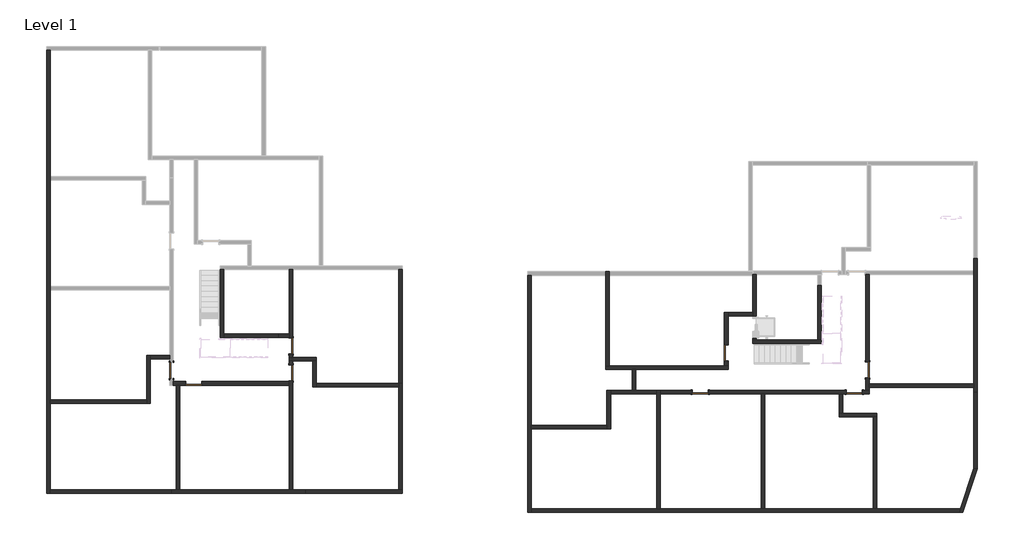
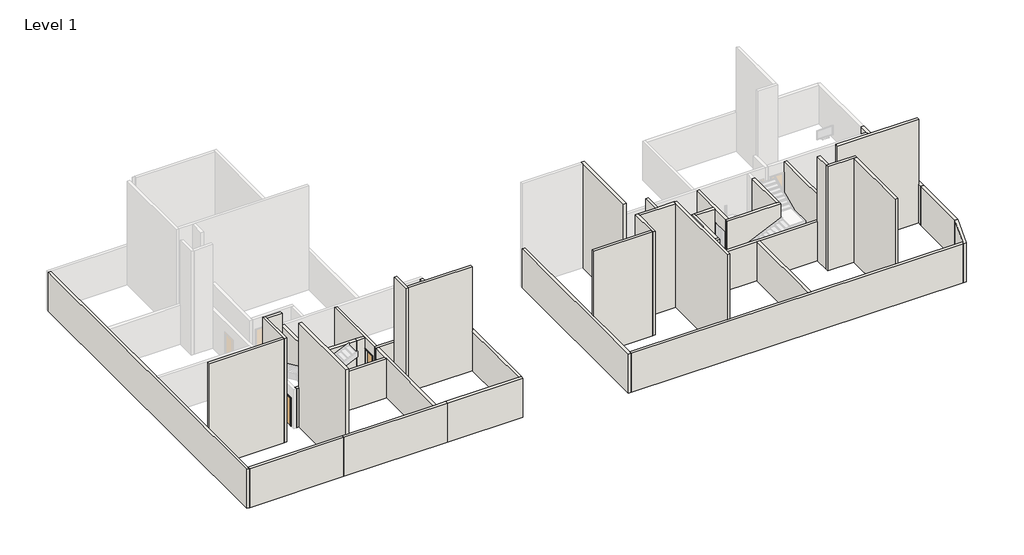
# One storey, part 1 of 2: 43 walls, 8 doors.
# Revit data of these elements (continued)
# Room, not placed, phase "New Construction", upper offset 0 cm, lower offset 0 cm
#   Number = "5"
#   Name = "Room"
# Room, not placed, phase "New Construction", upper offset 0 cm, lower offset 0 cm
#   Number = "6"
#   Name = "Room"
# Room at (-9476.825, 5160.6) mm, phase "New Construction", upper level "Level 1", upper offset 243.84 cm, lower offset 0 cm
#   Number = "124"
#   Name = "Room"
# Room, not placed, phase "New Construction", upper offset 0 cm, lower offset 0 cm
#   Number = "34"
#   Name = "Room"
# Room, not placed, phase "New Construction", upper offset 0 cm, lower offset 0 cm
#   Number = "35"
#   Name = "Room"
# Room, not placed, phase "New Construction", upper offset 0 cm, lower offset 0 cm
#   Number = "9"
#   Name = "Room"
# Room, not placed, phase "New Construction", upper offset 0 cm, lower offset 0 cm
#   Number = "10"
#   Name = "Room"
# Room, not placed, phase "New Construction", upper offset 0 cm, lower offset 0 cm
#   Number = "125"
#   Name = "Room"
# Room, not placed, phase "New Construction", upper offset 0 cm, lower offset 0 cm
#   Number = "126"
#   Name = "Room"
# Room, not placed, phase "New Construction", upper offset 0 cm, lower offset 0 cm
#   Number = "127"
#   Name = "Room"
# Room, not placed, phase "New Construction", upper offset 0 cm, lower offset 0 cm
#   Number = "128"
#   Name = "Room"
# Room, not placed, phase "New Construction", upper offset 0 cm, lower offset 0 cm
#   Number = "129"
#   Name = "Room"
# Room, not placed, phase "New Construction", upper offset 0 cm, lower offset 0 cm
#   Number = "91"
#   Name = "Room"
# Room at (-20321.225, 11202.195) mm, phase "New Construction", upper level "Level 1", upper offset 243.84 cm, lower offset 0 cm
#   Number = "130"
#   Name = "Room"
# Room at (-5594.466, -7580.79) mm, phase "New Construction", upper level "Level 1", upper offset 243.84 cm, lower offset 0 cm
#   Number = "131"
#   Name = "Room"
# Room at (-4954.966, -1430.614) mm, phase "New Construction", upper level "Level 1", upper offset 243.84 cm, lower offset 0 cm
#   Number = "132"
#   Name = "Room"
# Room at (-12237.947, 10302.814) mm, phase "New Construction", upper level "Level 1", upper offset 243.84 cm, lower offset 0 cm
#   Number = "133"
#   Name = "Room"
# Room, not placed, phase "New Construction", upper offset 0 cm, lower offset 0 cm
#   Number = ""
#   Name = ""
# Room, not placed, phase "New Construction", upper offset 0 cm, lower offset 0 cm
#   Number = "70"
#   Name = "Room"
# Room, not placed, phase "New Construction", upper offset 0 cm, lower offset 0 cm
#   Number = "71"
#   Name = "Room"
# Room, not placed, phase "New Construction", upper offset 0 cm, lower offset 0 cm
#   Number = "92"
#   Name = "Room"
# Room, not placed, phase "New Construction", upper offset 0 cm, lower offset 0 cm
#   Number = ""
#   Name = ""
# Room, not placed, phase "New Construction", upper offset 0 cm, lower offset 0 cm
#   Number = ""
#   Name = ""
# Room, not placed, phase "New Construction", upper offset 0 cm, lower offset 0 cm
#   Number = "37"
#   Name = "Room"
# Room, not placed, phase "New Construction", upper offset 0 cm, lower offset 0 cm
#   Number = ""
#   Name = "Banyo"
# Room, not placed, phase "New Construction", upper offset 0 cm, lower offset 0 cm
#   Number = ""
#   Name = ""
# Room, not placed, phase "New Construction", upper offset 0 cm, lower offset 0 cm
#   Number = ""
#   Name = "Yatak Odası"
# Room, not placed, phase "New Construction", upper offset 0 cm, lower offset 0 cm
#   Number = "39"
#   Name = "Room"
# Room, not placed, phase "New Construction", upper offset 0 cm, lower offset 0 cm
#   Number = ""
#   Name = "Salon-Mutfak"
# Area at (-11214.009, 13625.616) mm, upper offset 243.84 cm, lower offset 0 cm
#   Number = "9"
#   Name = "Area"
# Room, not placed, phase "New Construction", upper offset 0 cm, lower offset 0 cm
#   Number = "134"
#   Name = "Room"
# Room at (-19334.034, -2481.955) mm, phase "New Construction", upper level "Level 1", upper offset 243.84 cm, lower offset 0 cm
#   Number = "135"
#   Name = "Room"
# Room, not placed, phase "New Construction", upper offset 0 cm, lower offset 0 cm
#   Number = "40"
#   Name = "Room"
# Room, not placed, phase "New Construction", upper offset 0 cm, lower offset 0 cm
#   Number = "41"
#   Name = "Room"
# Area, not placed, upper offset 0 cm, lower offset 0 cm
#   Number = "8"
#   Name = "Dere Parsel Toplam Alan"
# Room, not placed, phase "New Construction", upper offset 0 cm, lower offset 0 cm
#   Number = "108"
#   Name = "ASANSÖR"
# Room, not placed, phase "New Construction", upper offset 0 cm, lower offset 0 cm
#   Number = "89"
#   Name = "Room"
# Room, not placed, phase "New Construction", upper offset 0 cm, lower offset 0 cm
#   Number = "19"
#   Name = "Room"
# Room, not placed, phase "New Construction", upper offset 0 cm, lower offset 0 cm
#   Number = ""
#   Name = ""
# Room, not placed, phase "New Construction", upper offset 0 cm, lower offset 0 cm
#   Number = "21"
#   Name = "Room"
# Room, not placed, phase "New Construction", upper offset 0 cm, lower offset 0 cm
#   Number = "22"
#   Name = "Room"
# Room, not placed, phase "New Construction", upper offset 0 cm, lower offset 0 cm
#   Number = "23"
#   Name = "Room"
# Room, not placed, phase "New Construction", upper offset 0 cm, lower offset 0 cm
#   Number = "24"
#   Name = "Room"
# Room, not placed, phase "New Construction", upper offset 0 cm, lower offset 0 cm
#   Number = "25"
#   Name = "Room"
# Room, not placed, phase "New Construction", upper offset 0 cm, lower offset 0 cm
#   Number = "64"
#   Name = "Room"
# Room, not placed, phase "New Construction", upper offset 0 cm, lower offset 0 cm
#   Number = "65"
#   Name = "Room"
# Room, not placed, phase "New Construction", upper offset 0 cm, lower offset 0 cm
#   Number = "66"
#   Name = "Room"
# Room, not placed, phase "New Construction", upper offset 0 cm, lower offset 0 cm
#   Number = ""
#   Name = ""
# Room, not placed, phase "New Construction", upper offset 0 cm, lower offset 0 cm
#   Number = "27"
#   Name = "Room"
# Room, not placed, phase "New Construction", upper offset 0 cm, lower offset 0 cm
#   Number = "42"
#   Name = "Room"
# Area, not placed, upper offset 0 cm, lower offset 0 cm
#   Number = "2"
#   Name = "Area"
# Room, not placed, phase "New Construction", upper offset 0 cm, lower offset 0 cm
#   Number = "43"
#   Name = "Room"
# Room, not placed, phase "New Construction", upper offset 0 cm, lower offset 0 cm
#   Number = ""
#   Name = ""
# Room, not placed, phase "New Construction", upper offset 0 cm, lower offset 0 cm
#   Number = "94"
#   Name = "Room"
# Room, not placed, phase "New Construction", upper offset 0 cm, lower offset 0 cm
#   Number = ""
#   Name = ""
# Room at (-18935.383, 3898.657) mm, phase "New Construction", upper level "Level 1", upper offset 243.84 cm, lower offset 0 cm
#   Number = "136"
#   Name = "Room"
# Room, not placed, phase "New Construction", upper offset 0 cm, lower offset 0 cm
#   Number = "1"
#   Name = "Room"
# Area, not placed, upper offset 0 cm, lower offset 0 cm
#   Number = "3"
#   Name = "Area"
# Room, not placed, phase "New Construction", upper offset 0 cm, lower offset 0 cm
#   Number = "7"
#   Name = "Room"
# Room, not placed, phase "New Construction", upper offset 0 cm, lower offset 0 cm
#   Number = "8"
#   Name = "Room"
# Room, not placed, phase "New Construction", upper offset 0 cm, lower offset 0 cm
#   Number = "2"
#   Name = "Room"
# Room, not placed, phase "New Construction", upper offset 0 cm, lower offset 0 cm
#   Number = "46"
#   Name = "Room"
# Room, not placed, phase "New Construction", upper offset 0 cm, lower offset 0 cm
#   Number = "3"
#   Name = "Room"
# Room, not placed, phase "New Construction", upper offset 0 cm, lower offset 0 cm
#   Number = ""
#   Name = ""
# Room, not placed, phase "New Construction", upper offset 0 cm, lower offset 0 cm
#   Number = "4"
#   Name = "Room"
# Area, not placed, upper offset 0 cm, lower offset 0 cm
#   Number = "1"
#   Name = "Area"
# Room, not placed, phase "New Construction", upper offset 0 cm, lower offset 0 cm
#   Number = ""
#   Name = ""
# Room, not placed, phase "New Construction", upper offset 0 cm, lower offset 0 cm
#   Number = "29"
#   Name = "Room"
# Area, not placed, upper offset 0 cm, lower offset 0 cm
#   Number = "7"
#   Name = "Dere Parsel Toplam Alan"
# Room, not placed, phase "New Construction", upper offset 0 cm, lower offset 0 cm
#   Number = "95"
#   Name = "ASANSÖR"
# Room, not placed, phase "New Construction", upper offset 0 cm, lower offset 0 cm
#   Number = "96"
#   Name = "Room"
# Room, not placed, phase "New Construction", upper offset 0 cm, lower offset 0 cm
#   Number = "97"
#   Name = "7"
# Room, not placed, phase "New Construction", upper offset 0 cm, lower offset 0 cm
#   Number = "98"
#   Name = "8"
# Room, not placed, phase "New Construction", upper offset 0 cm, lower offset 0 cm
#   Number = "99"
#   Name = "9"
# Room, not placed, phase "New Construction", upper offset 0 cm, lower offset 0 cm
#   Number = "100"
#   Name = "1"
# Room, not placed, phase "New Construction", upper offset 0 cm, lower offset 0 cm
#   Number = "101"
#   Name = "5"
# Room, not placed, phase "New Construction", upper offset 0 cm, lower offset 0 cm
#   Number = "102"
#   Name = "2"
# Room, not placed, phase "New Construction", upper offset 0 cm, lower offset 0 cm
#   Number = "103"
#   Name = "4"
# Room, not placed, phase "New Construction", upper offset 0 cm, lower offset 0 cm
#   Number = "104"
#   Name = "3"
# Room, not placed, phase "New Construction", upper offset 0 cm, lower offset 0 cm
#   Number = "105"
#   Name = "6"
